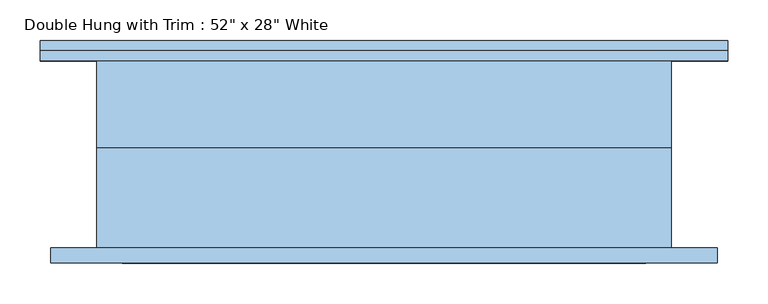
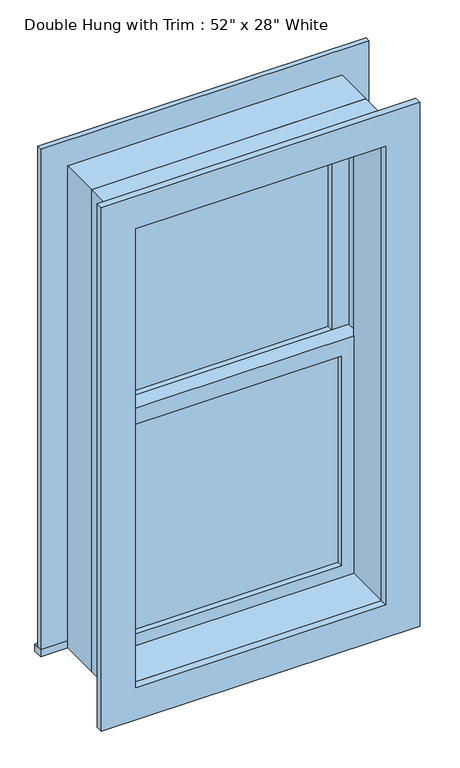
"""IFC4 building model written with IfcOpenShell, lengths in millimetres: window geometry."""

import ifcopenshell
import ifcopenshell.guid

model = None  # the IFC model being written
_history = None  # IfcOwnerHistory: only IFC2X3 demands one
_inside = {}  # id of a spatial element -> (the spatial element, [elements in it])
_under = {}  # id of a project, library or spatial element -> (it, [spatial elements below it])
_declared = {}  # id of a project -> (the project, [libraries it declares])
_typed = {}  # id of a type object -> (the type object, [elements of that type])
_made_of = {}  # id of a material, layer set ... -> (it, [elements and type objects made of it])


def new_model(schema):
    """Start an empty IFC model of exactly this schema.

    Asked for "IFC4X3", IfcOpenShell would pick the latest addendum, in which some entities
    have other attributes; the version numbers below select the first issue.
    IFC2X3 requires an IfcOwnerHistory on every rooted entity: one is made here for all.
    """
    global model, _history
    if schema == "IFC4X3":
        model = ifcopenshell.file(schema_version=(4, 3, 0, 0))
    else:
        model = ifcopenshell.file(schema=schema)
    _inside.clear()
    _under.clear()
    _declared.clear()
    _typed.clear()
    _made_of.clear()
    _history = None
    if model.schema == "IFC2X3":
        org = make("IfcOrganization", Name="unknown")
        user = make(
            "IfcPersonAndOrganization",
            ThePerson=make("IfcPerson", FamilyName="unknown"),
            TheOrganization=org,
        )
        app = make(
            "IfcApplication",
            ApplicationDeveloper=org,
            Version="unknown",
            ApplicationFullName="unknown",
            ApplicationIdentifier="unknown",
        )
        _history = make(
            "IfcOwnerHistory",
            OwningUser=user,
            OwningApplication=app,
            ChangeAction="ADDED",
            CreationDate=0,
        )
    return model


def make(cls, **values):
    """One entity of the class cls with the attributes given. An attribute that is None is left unset."""
    return model.create_entity(
        cls, **{name: value for name, value in values.items() if value is not None}
    )


def rooted(cls, **values):
    """An entity with a GlobalId (a new one), such as an element, a storey or a relation."""
    return make(cls, GlobalId=ifcopenshell.guid.new(), OwnerHistory=_history, **values)


def si_unit(unit_type, name, prefix=None):
    """IfcSIUnit, for example si_unit("LENGTHUNIT", "METRE", prefix="MILLI")."""
    return make("IfcSIUnit", UnitType=unit_type, Prefix=prefix, Name=name)


def assignment(units):
    """IfcUnitAssignment: the units of a project."""
    return None if units is None else make("IfcUnitAssignment", Units=units)


def point(xyz):
    """IfcCartesianPoint."""
    return None if xyz is None else make("IfcCartesianPoint", Coordinates=xyz)


def direction(xyz):
    """IfcDirection."""
    return None if xyz is None else make("IfcDirection", DirectionRatios=xyz)


def frame(location, z_axis=None, x_axis=None):
    """IfcAxis2Placement3D, a coordinate frame: its origin and axes. An axis left out is left unset."""
    return make(
        "IfcAxis2Placement3D",
        Location=point(location),
        Axis=direction(z_axis),
        RefDirection=direction(x_axis),
    )


def origin():
    """The frame at (0, 0, 0) with its axes left unset."""
    return frame((0.0, 0.0, 0.0))


def place(relative_to, where):
    """IfcLocalPlacement: puts the frame where relative to a parent placement (None: the world)."""
    return make(
        "IfcLocalPlacement", PlacementRelTo=relative_to, RelativePlacement=where
    )


def context(
    kind, dimensions, precision=None, world=None, true_north=None, identifier=None
):
    """IfcGeometricRepresentationContext, for example the 3D "Model" context."""
    return make(
        "IfcGeometricRepresentationContext",
        ContextIdentifier=identifier,
        ContextType=kind,
        CoordinateSpaceDimension=dimensions,
        Precision=precision,
        WorldCoordinateSystem=world,
        TrueNorth=true_north,
    )


def project(units=None, contexts=None):
    """IfcProject with its units and contexts."""
    return rooted(
        "IfcProject",
        Name="project",
        RepresentationContexts=contexts,
        UnitsInContext=assignment(units),
    )


def spatial(cls, under=None, at=None, **own):
    """A site, building, storey or space (cls), placed at a placement, below another one or the project."""
    s = rooted(cls, ObjectPlacement=at, **own)
    if under is not None:
        _under.setdefault(under.id(), (under, []))[1].append(s)
    return s


def polyline(points):
    """IfcPolyline through the points."""
    return make("IfcPolyline", Points=[point(p) for p in points])


def outline(outer, holes=None, kind="AREA"):
    """IfcArbitraryClosedProfileDef: a profile drawn as a closed curve; with holes, ...WithVoids."""
    if holes is None:
        return make("IfcArbitraryClosedProfileDef", ProfileType=kind, OuterCurve=outer)
    return make(
        "IfcArbitraryProfileDefWithVoids",
        ProfileType=kind,
        OuterCurve=outer,
        InnerCurves=holes,
    )


def extrude(swept, where, along, depth):
    """IfcExtrudedAreaSolid: the profile swept, set in the frame where, extruded along a direction by depth."""
    return make(
        "IfcExtrudedAreaSolid",
        SweptArea=swept,
        Position=where,
        ExtrudedDirection=direction(along),
        Depth=depth,
    )


def shape(context_of_items, identifier, shape_type, items):
    """IfcShapeRepresentation: the items that make up one representation, for example the "Body"."""
    return make(
        "IfcShapeRepresentation",
        ContextOfItems=context_of_items,
        RepresentationIdentifier=identifier,
        RepresentationType=shape_type,
        Items=items,
    )


def source(mapping_origin, context_of_items, identifier, shape_type, items):
    """IfcRepresentationMap: a shape defined once, which mapped items show again and again."""
    return make(
        "IfcRepresentationMap",
        MappingOrigin=mapping_origin,
        MappedRepresentation=shape(context_of_items, identifier, shape_type, items),
    )


def transform(
    local_origin,
    x_axis=None,
    y_axis=None,
    z_axis=None,
    scale=None,
    scale2=None,
    scale3=None,
    uniform=True,
):
    """IfcCartesianTransformationOperator3D, or its non-uniform kind. x_axis, y_axis, z_axis: its Axis1, 2, 3."""
    if uniform:
        return make(
            "IfcCartesianTransformationOperator3D",
            Axis1=direction(x_axis),
            Axis2=direction(y_axis),
            LocalOrigin=point(local_origin),
            Scale=scale,
            Axis3=direction(z_axis),
        )
    return make(
        "IfcCartesianTransformationOperator3DnonUniform",
        Axis1=direction(x_axis),
        Axis2=direction(y_axis),
        LocalOrigin=point(local_origin),
        Scale=scale,
        Axis3=direction(z_axis),
        Scale2=scale2,
        Scale3=scale3,
    )


def mapped(mapping_source, mapping_target):
    """IfcMappedItem: shows the shape of a source again, moved by a transform."""
    return make(
        "IfcMappedItem", MappingSource=mapping_source, MappingTarget=mapping_target
    )


def made_of(thing, what):
    """Note that an element or type object is made of a material, layer set ...; save() writes the relation."""
    if what is not None:
        _made_of.setdefault(what.id(), (what, []))[1].append(thing)
    return thing


def element(
    cls,
    number,
    at=None,
    inside=None,
    cuts=None,
    type_object=None,
    material=None,
    context=None,
    identifier="Body",
    shape_type=None,
    held_by="IfcProductDefinitionShape",
    body=None,
    shapes=None,
    **own,
):
    """One element of the class cls, such as IfcWall. Its Tag is "e" and its number.

    at: its placement. inside: the storey or other place that contains it. cuts: it is an
    opening in that element (IfcRelVoidsElement). A single representation is given by context,
    identifier, shape_type and body (its items); several are given by shapes. held_by: the class
    of the entity that holds the representations. save() writes the other relations.
    """
    e = rooted(cls, Tag="e%d" % number, ObjectPlacement=at, **own)
    if body is not None:
        shapes = [shape(context, identifier, shape_type, body)]
    if shapes is not None:
        e.Representation = make(held_by, Representations=shapes)
    if inside is not None:
        _inside.setdefault(inside.id(), (inside, []))[1].append(e)
    if cuts is not None:
        rooted(
            "IfcRelVoidsElement", RelatingBuildingElement=cuts, RelatedOpeningElement=e
        )
    if type_object is not None:
        _typed.setdefault(type_object.id(), (type_object, []))[1].append(e)
    return made_of(e, material)


def aggregate(whole, parts):
    """IfcRelAggregates: a whole, such as a stair, and the parts it consists of."""
    return rooted("IfcRelAggregates", RelatingObject=whole, RelatedObjects=parts)


def save(model, path):
    """Write the relations noted so far, then the file.

    IfcRelAggregates (storeys below a building ...), IfcRelContainedInSpatialStructure (elements
    in a storey), IfcRelDefinesByType, IfcRelAssociatesMaterial and IfcRelDeclares: one each for
    every whole, place, type object, material and project.
    """
    for whole, parts in _under.values():
        aggregate(whole, parts)
    for where, things in _inside.values():
        rooted(
            "IfcRelContainedInSpatialStructure",
            RelatedElements=things,
            RelatingStructure=where,
        )
    for kind, things in _typed.values():
        rooted("IfcRelDefinesByType", RelatedObjects=things, RelatingType=kind)
    for what, things in _made_of.values():
        rooted("IfcRelAssociatesMaterial", RelatedObjects=things, RelatingMaterial=what)
    for by, libraries in _declared.values():
        rooted("IfcRelDeclares", RelatingContext=by, RelatedDefinitions=libraries)
    model.write(path)


def window_fffe74c7(model_context):
    return source(origin(), model_context, "Body", "SweptSolid", [
        extrude(outline(polyline([(-292.1, 36.5125008), (292.1, 36.5125008), (292.1, 23.8125008), (-292.1, 23.8125008), (-292.1, 36.5125008)])), frame((0.0, 0.0, 571.5), z_axis=(0.0, 0.0, 1.0), x_axis=(1.0, 0.0, 0.0)), (0.0, 0.0, 1.0), 574.675),
        extrude(outline(polyline([(1190.625, -336.55), (527.05, -336.55), (527.05, 336.55), (1190.625, 336.55), (1190.625, -336.55)]), holes=[polyline([(1146.175, -292.1), (1146.175, 292.1), (571.5, 292.1), (571.5, -292.1), (1146.175, -292.1)])]), frame((0.0, 7.9375008, 0.0), z_axis=(0.0, 1.0, 0.0), x_axis=(0.0, 0.0, 1.0)), (0.0, 0.0, 1.0), 44.45),
        extrude(outline(polyline([(-425.45, 141.2875008), (425.45, 141.2875008), (425.45, 115.8875008), (-425.45, 115.8875008), (-425.45, 141.2875008)])), frame((0.0, 0.0, 508.0), z_axis=(0.0, 0.0, 1.0), x_axis=(1.0, 0.0, 0.0)), (0.0, 0.0, 1.0), 19.05),
        extrude(outline(polyline([(1809.75, -336.55), (1809.75, 336.55), (527.05, 336.55), (527.05, 425.45), (1898.65, 425.45), (1898.65, -425.45), (527.05, -425.45), (527.05, -336.55), (1809.75, -336.55)])), frame((0.0, 115.8875008, 0.0), z_axis=(0.0, 1.0, 0.0), x_axis=(0.0, 0.0, 1.0)), (0.0, 0.0, 1.0), 12.7),
        extrude(outline(polyline([(1885.95, 412.75), (1885.95, -412.75), (450.85, -412.75), (450.85, 412.75), (1885.95, 412.75)]), holes=[polyline([(1797.05, 323.85), (539.75, 323.85), (539.75, -323.85), (1797.05, -323.85), (1797.05, 323.85)])]), frame((0.0, -134.9375008, 0.0), z_axis=(0.0, 1.0, 0.0), x_axis=(0.0, 0.0, 1.0)), (0.0, 0.0, 1.0), 19.05),
        extrude(outline(polyline([(292.1, 68.2625008), (-292.1, 68.2625008), (-292.1, 80.9625008), (292.1, 80.9625008), (292.1, 68.2625008)])), frame((0.0, 0.0, 1190.625), z_axis=(0.0, 0.0, 1.0), x_axis=(1.0, 0.0, 0.0)), (0.0, 0.0, 1.0), 574.675),
        extrude(outline(polyline([(1809.75, -336.55), (1146.175, -336.55), (1146.175, 336.55), (1809.75, 336.55), (1809.75, -336.55)]), holes=[polyline([(1765.3, -292.1), (1765.3, 292.1), (1190.625, 292.1), (1190.625, -292.1), (1765.3, -292.1)])]), frame((0.0, 52.3875008, 0.0), z_axis=(0.0, 1.0, 0.0), x_axis=(0.0, 0.0, 1.0)), (0.0, 0.0, 1.0), 44.45),
        extrude(outline(polyline([(1828.8, -355.6), (508.0, -355.6), (508.0, 355.6), (1828.8, 355.6), (1828.8, -355.6)]), holes=[polyline([(1797.05, -323.85), (1797.05, 323.85), (539.75, 323.85), (539.75, -323.85), (1797.05, -323.85)])]), frame((0.0, -115.8875008, 0.0), z_axis=(0.0, 1.0, 0.0), x_axis=(0.0, 0.0, 1.0)), (0.0, 0.0, 1.0), 123.8250015),
        extrude(outline(polyline([(1828.8, 355.6), (1828.8, -355.6), (508.0, -355.6), (508.0, 355.6), (1828.8, 355.6)]), holes=[polyline([(1809.75, 336.55), (527.05, 336.55), (527.05, -336.55), (1809.75, -336.55), (1809.75, 336.55)])]), frame((0.0, 7.9375008, 0.0), z_axis=(0.0, 1.0, 0.0), x_axis=(0.0, 0.0, 1.0)), (0.0, 0.0, 1.0), 107.95),
    ])


if __name__ == "__main__":
    model = new_model("IFC4")
    model_context = context("Model", 3, world=origin())
    ifc_project = project(units=[si_unit("LENGTHUNIT", "METRE", prefix="MILLI")], contexts=[model_context])
    site = spatial("IfcSite", under=ifc_project)
    building = spatial("IfcBuilding", under=site)
    placement = place(None, origin())
    window_shape = window_fffe74c7(model_context)
    element("IfcWindow", 1, ObjectType="Double Hung with Trim : 52\" x 28\" White", at=placement, inside=building, context=model_context, shape_type="MappedRepresentation", body=[
        mapped(window_shape, transform((0.0, 0.0, 0.0), x_axis=(1.0, 0.0, 0.0), y_axis=(0.0, 1.0, 0.0), z_axis=(0.0, 0.0, 1.0))),
    ])
    save(model, "model.ifc")

# Revit data of these elements
# Type "Double Hung with Trim : 52\" x 28\" White"
#   Type Mark = "80"
#   Construction Type Id = "GSP4R"
#   Assembly Code = "B2020100"
#   Analytic Construction = "1/8 in Pilkington single glazing"
#   Visual Light Transmittance = 0.9
#   Solar Heat Gain Coefficient = 0.78
#   Heat Transfer Coefficient (U) = 3.6886 W/(m²·K)
#   Height = 4' - 4"
#   Default Sill Height = 1' - 8"
#   Trim Projection - Ext. = 0' - 0 1/2"
#   Trim Projection - Int. = 0' - 0 3/4"
#   Trim Width - Exterior = 0' - 3 1/2"
#   Trim Width - Interior = 0' - 3 1/2"
#   Width = 2' - 4"
#   Window Inset = 0' - 0 3/4"
#   COBie.Type = no
#   Glass Pane Material = Glass
#   Sash Material = Sash - White
#   Trim Exterior Material = Trim - White
#   Trim Interior Material = Trim - White
#   Wall Closure = (empty or 0)
# Element 1 (IfcWindow, "Double Hung with Trim : 52\" x 28\" White")
#   Materials on its faces: "Sash - White", "Trim - White", "Glass"
# Materials
#   "Glass": class "Glass", colour RGB 0 128 192, transparency 0.75, Description = "Soda Lime Glass", Cost = 0
#   "Sash - White": class "Wood", colour RGB 255 255 255, transparency 0, Cost = 0
#   "Trim - White": class "Wood", colour RGB 255 255 255, transparency 0, Cost = 0
